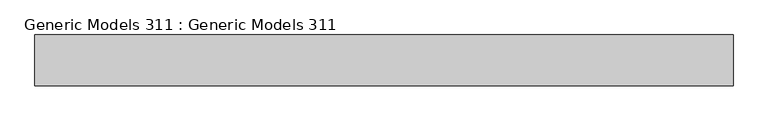
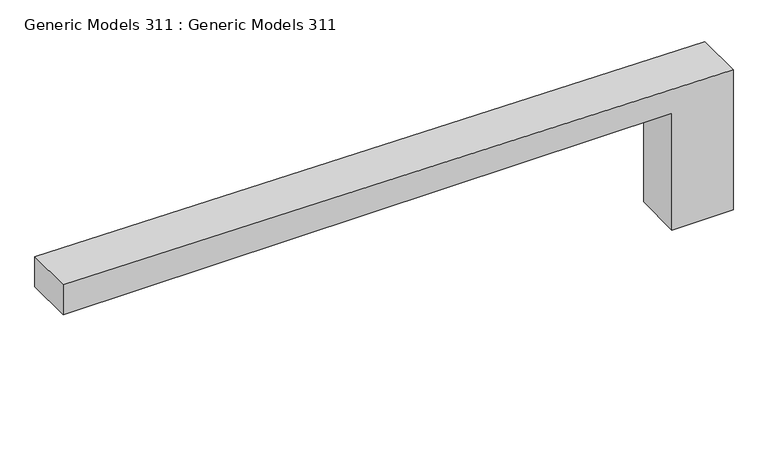
"""IFC4 building model written with IfcOpenShell, lengths in millimetres: proxy geometry, Generic Models 311 : Generic Models 311."""

from ifc_helpers import new_model, si_unit, frame, origin, place, context, project, spatial, polyline, outline, extrude, source, transform, mapped, element, save


def generic_models_311_generic_models_311_b86710ee(model_context):
    return source(origin(), model_context, "Body", "SweptSolid", [
        extrude(outline(polyline([(123799.346, 4406.7263704), (123602.496, 4406.7263704), (123602.496, 8191.3263705), (122834.5072951, 8191.3263705), (122834.5072951, 8572.3263705), (123755.1653939, 8572.3263705), (123799.346, 4406.7263704)])), frame((0.0, -4109.6428838, 0.0), z_axis=(0.0, 1.0, 0.0), x_axis=(0.0, 0.0, 1.0)), (0.0, 0.0, 1.0), 304.8),
    ])


if __name__ == "__main__":
    model = new_model("IFC4")
    model_context = context("Model", 3, world=origin())
    ifc_project = project(units=[si_unit("LENGTHUNIT", "METRE", prefix="MILLI")], contexts=[model_context])
    site = spatial("IfcSite", under=ifc_project)
    building = spatial("IfcBuilding", under=site)
    placement = place(None, origin())
    generic_models_311_generic_models_311_shape = generic_models_311_generic_models_311_b86710ee(model_context)
    element("IfcBuildingElementProxy", 1, Name="Generic Models 311 : Generic Models 311", ObjectType="Generic Models 311 : Generic Models 311", at=placement, inside=building, context=model_context, shape_type="MappedRepresentation", body=[
        mapped(generic_models_311_generic_models_311_shape, transform((0.0, 0.0, 0.0), x_axis=(1.0, 0.0, 0.0), y_axis=(0.0, 1.0, 0.0), z_axis=(0.0, 0.0, 1.0))),
    ])
    save(model, "model.ifc")

# Revit data of these elements
# Element 1 (IfcBuildingElementProxy, "Generic Models 311 : Generic Models 311")
#   Materials on its faces: "_CONCRETE SLAB W/ WIRE MESH (SEE STRUCT. DWGS) - SLOPE 1% AWAY FROM BUILDING"
# Materials
#   "_CONCRETE SLAB W/ WIRE MESH (SEE STRUCT. DWGS) - SLOPE 1% AWAY FROM BUILDING": class "Generic", colour RGB 191 191 191, transparency 0, Cost = 0
